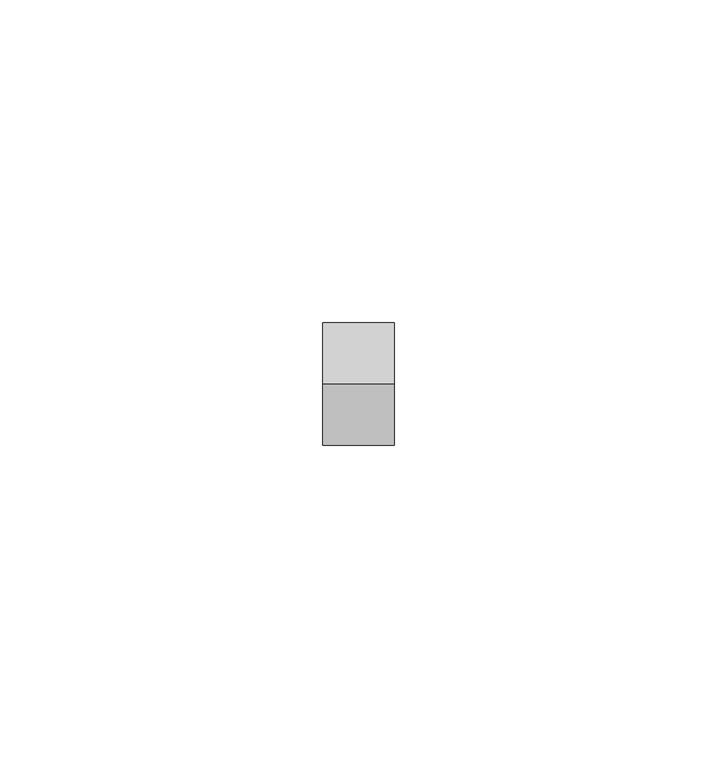
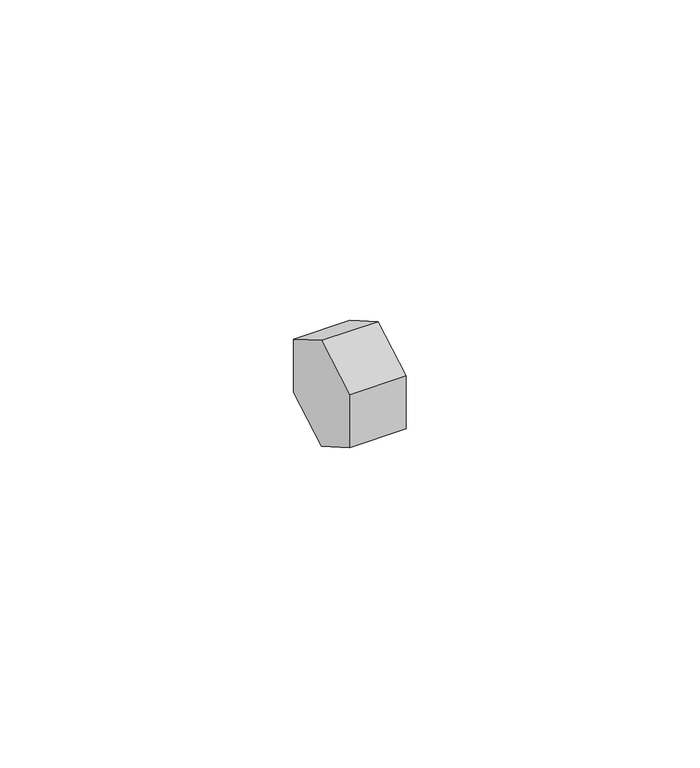
"""IFC4 building model written with IfcOpenShell, lengths in millimetres: proxy geometry, Generic Models 7:Generic Models 1:8:Generic Models 1:8 : Generic Models 7:Generic Models 1:337419:58 : Generic Models 7:Generic Models 1:8:Generic Models 1:8 : Generic Models 7:Generic Models 1:337419:315935."""

import ifcopenshell
import ifcopenshell.guid

model = None  # the IFC model being written
_history = None  # IfcOwnerHistory: only IFC2X3 demands one
_inside = {}  # id of a spatial element -> (the spatial element, [elements in it])
_under = {}  # id of a project, library or spatial element -> (it, [spatial elements below it])
_declared = {}  # id of a project -> (the project, [libraries it declares])
_typed = {}  # id of a type object -> (the type object, [elements of that type])
_made_of = {}  # id of a material, layer set ... -> (it, [elements and type objects made of it])


def new_model(schema):
    """Start an empty IFC model of exactly this schema.

    Asked for "IFC4X3", IfcOpenShell would pick the latest addendum, in which some entities
    have other attributes; the version numbers below select the first issue.
    IFC2X3 requires an IfcOwnerHistory on every rooted entity: one is made here for all.
    """
    global model, _history
    if schema == "IFC4X3":
        model = ifcopenshell.file(schema_version=(4, 3, 0, 0))
    else:
        model = ifcopenshell.file(schema=schema)
    _inside.clear()
    _under.clear()
    _declared.clear()
    _typed.clear()
    _made_of.clear()
    _history = None
    if model.schema == "IFC2X3":
        org = make("IfcOrganization", Name="unknown")
        user = make(
            "IfcPersonAndOrganization",
            ThePerson=make("IfcPerson", FamilyName="unknown"),
            TheOrganization=org,
        )
        app = make(
            "IfcApplication",
            ApplicationDeveloper=org,
            Version="unknown",
            ApplicationFullName="unknown",
            ApplicationIdentifier="unknown",
        )
        _history = make(
            "IfcOwnerHistory",
            OwningUser=user,
            OwningApplication=app,
            ChangeAction="ADDED",
            CreationDate=0,
        )
    return model


def make(cls, **values):
    """One entity of the class cls with the attributes given. An attribute that is None is left unset."""
    return model.create_entity(
        cls, **{name: value for name, value in values.items() if value is not None}
    )


def rooted(cls, **values):
    """An entity with a GlobalId (a new one), such as an element, a storey or a relation."""
    return make(cls, GlobalId=ifcopenshell.guid.new(), OwnerHistory=_history, **values)


def si_unit(unit_type, name, prefix=None):
    """IfcSIUnit, for example si_unit("LENGTHUNIT", "METRE", prefix="MILLI")."""
    return make("IfcSIUnit", UnitType=unit_type, Prefix=prefix, Name=name)


def assignment(units):
    """IfcUnitAssignment: the units of a project."""
    return None if units is None else make("IfcUnitAssignment", Units=units)


def point(xyz):
    """IfcCartesianPoint."""
    return None if xyz is None else make("IfcCartesianPoint", Coordinates=xyz)


def direction(xyz):
    """IfcDirection."""
    return None if xyz is None else make("IfcDirection", DirectionRatios=xyz)


def frame(location, z_axis=None, x_axis=None):
    """IfcAxis2Placement3D, a coordinate frame: its origin and axes. An axis left out is left unset."""
    return make(
        "IfcAxis2Placement3D",
        Location=point(location),
        Axis=direction(z_axis),
        RefDirection=direction(x_axis),
    )


def origin():
    """The frame at (0, 0, 0) with its axes left unset."""
    return frame((0.0, 0.0, 0.0))


def place(relative_to, where):
    """IfcLocalPlacement: puts the frame where relative to a parent placement (None: the world)."""
    return make(
        "IfcLocalPlacement", PlacementRelTo=relative_to, RelativePlacement=where
    )


def context(
    kind, dimensions, precision=None, world=None, true_north=None, identifier=None
):
    """IfcGeometricRepresentationContext, for example the 3D "Model" context."""
    return make(
        "IfcGeometricRepresentationContext",
        ContextIdentifier=identifier,
        ContextType=kind,
        CoordinateSpaceDimension=dimensions,
        Precision=precision,
        WorldCoordinateSystem=world,
        TrueNorth=true_north,
    )


def project(units=None, contexts=None):
    """IfcProject with its units and contexts."""
    return rooted(
        "IfcProject",
        Name="project",
        RepresentationContexts=contexts,
        UnitsInContext=assignment(units),
    )


def spatial(cls, under=None, at=None, **own):
    """A site, building, storey or space (cls), placed at a placement, below another one or the project."""
    s = rooted(cls, ObjectPlacement=at, **own)
    if under is not None:
        _under.setdefault(under.id(), (under, []))[1].append(s)
    return s


def polyline(points):
    """IfcPolyline through the points."""
    return make("IfcPolyline", Points=[point(p) for p in points])


def outline(outer, holes=None, kind="AREA"):
    """IfcArbitraryClosedProfileDef: a profile drawn as a closed curve; with holes, ...WithVoids."""
    if holes is None:
        return make("IfcArbitraryClosedProfileDef", ProfileType=kind, OuterCurve=outer)
    return make(
        "IfcArbitraryProfileDefWithVoids",
        ProfileType=kind,
        OuterCurve=outer,
        InnerCurves=holes,
    )


def extrude(swept, where, along, depth):
    """IfcExtrudedAreaSolid: the profile swept, set in the frame where, extruded along a direction by depth."""
    return make(
        "IfcExtrudedAreaSolid",
        SweptArea=swept,
        Position=where,
        ExtrudedDirection=direction(along),
        Depth=depth,
    )


def shape(context_of_items, identifier, shape_type, items):
    """IfcShapeRepresentation: the items that make up one representation, for example the "Body"."""
    return make(
        "IfcShapeRepresentation",
        ContextOfItems=context_of_items,
        RepresentationIdentifier=identifier,
        RepresentationType=shape_type,
        Items=items,
    )


def source(mapping_origin, context_of_items, identifier, shape_type, items):
    """IfcRepresentationMap: a shape defined once, which mapped items show again and again."""
    return make(
        "IfcRepresentationMap",
        MappingOrigin=mapping_origin,
        MappedRepresentation=shape(context_of_items, identifier, shape_type, items),
    )


def transform(
    local_origin,
    x_axis=None,
    y_axis=None,
    z_axis=None,
    scale=None,
    scale2=None,
    scale3=None,
    uniform=True,
):
    """IfcCartesianTransformationOperator3D, or its non-uniform kind. x_axis, y_axis, z_axis: its Axis1, 2, 3."""
    if uniform:
        return make(
            "IfcCartesianTransformationOperator3D",
            Axis1=direction(x_axis),
            Axis2=direction(y_axis),
            LocalOrigin=point(local_origin),
            Scale=scale,
            Axis3=direction(z_axis),
        )
    return make(
        "IfcCartesianTransformationOperator3DnonUniform",
        Axis1=direction(x_axis),
        Axis2=direction(y_axis),
        LocalOrigin=point(local_origin),
        Scale=scale,
        Axis3=direction(z_axis),
        Scale2=scale2,
        Scale3=scale3,
    )


def mapped(mapping_source, mapping_target):
    """IfcMappedItem: shows the shape of a source again, moved by a transform."""
    return make(
        "IfcMappedItem", MappingSource=mapping_source, MappingTarget=mapping_target
    )


def made_of(thing, what):
    """Note that an element or type object is made of a material, layer set ...; save() writes the relation."""
    if what is not None:
        _made_of.setdefault(what.id(), (what, []))[1].append(thing)
    return thing


def element(
    cls,
    number,
    at=None,
    inside=None,
    cuts=None,
    type_object=None,
    material=None,
    context=None,
    identifier="Body",
    shape_type=None,
    held_by="IfcProductDefinitionShape",
    body=None,
    shapes=None,
    **own,
):
    """One element of the class cls, such as IfcWall. Its Tag is "e" and its number.

    at: its placement. inside: the storey or other place that contains it. cuts: it is an
    opening in that element (IfcRelVoidsElement). A single representation is given by context,
    identifier, shape_type and body (its items); several are given by shapes. held_by: the class
    of the entity that holds the representations. save() writes the other relations.
    """
    e = rooted(cls, Tag="e%d" % number, ObjectPlacement=at, **own)
    if body is not None:
        shapes = [shape(context, identifier, shape_type, body)]
    if shapes is not None:
        e.Representation = make(held_by, Representations=shapes)
    if inside is not None:
        _inside.setdefault(inside.id(), (inside, []))[1].append(e)
    if cuts is not None:
        rooted(
            "IfcRelVoidsElement", RelatingBuildingElement=cuts, RelatedOpeningElement=e
        )
    if type_object is not None:
        _typed.setdefault(type_object.id(), (type_object, []))[1].append(e)
    return made_of(e, material)


def aggregate(whole, parts):
    """IfcRelAggregates: a whole, such as a stair, and the parts it consists of."""
    return rooted("IfcRelAggregates", RelatingObject=whole, RelatedObjects=parts)


def save(model, path):
    """Write the relations noted so far, then the file.

    IfcRelAggregates (storeys below a building ...), IfcRelContainedInSpatialStructure (elements
    in a storey), IfcRelDefinesByType, IfcRelAssociatesMaterial and IfcRelDeclares: one each for
    every whole, place, type object, material and project.
    """
    for whole, parts in _under.values():
        aggregate(whole, parts)
    for where, things in _inside.values():
        rooted(
            "IfcRelContainedInSpatialStructure",
            RelatedElements=things,
            RelatingStructure=where,
        )
    for kind, things in _typed.values():
        rooted("IfcRelDefinesByType", RelatedObjects=things, RelatingType=kind)
    for what, things in _made_of.values():
        rooted("IfcRelAssociatesMaterial", RelatedObjects=things, RelatingMaterial=what)
    for by, libraries in _declared.values():
        rooted("IfcRelDeclares", RelatingContext=by, RelatedDefinitions=libraries)
    model.write(path)


def generic_models_35fd506f(model_context):
    return source(origin(), model_context, "Body", "SweptSolid", [
        extrude(outline(polyline([(-564915.9326015, 8757.3782009), (-564925.4576015, 8762.8774622), (-564925.4576015, 8773.8759848), (-564915.9326015, 8779.3752461), (-564906.4076015, 8773.8759848), (-564906.4076015, 8762.8774622), (-564915.9326015, 8757.3782009)])), frame((593804.563286, 0.0, 0.0), z_axis=(1.0, 0.0, 0.0), x_axis=(0.0, 1.0, 0.0)), (0.0, 0.0, 1.0), 11.1125),
    ])


if __name__ == "__main__":
    model = new_model("IFC4")
    model_context = context("Model", 3, world=origin())
    ifc_project = project(units=[si_unit("LENGTHUNIT", "METRE", prefix="MILLI")], contexts=[model_context])
    site = spatial("IfcSite", under=ifc_project)
    building = spatial("IfcBuilding", under=site)
    placement = place(None, origin())
    generic_models_shape = generic_models_35fd506f(model_context)
    element("IfcBuildingElementProxy", 1, Name="Generic Models 7:Generic Models 1:8:Generic Models 1:8 : Generic Models 7:Generic Models 1:337419:58 : Generic Models 7:Generic Models 1:8:Generic Models 1:8 : Generic Models 7:Generic Models 1:337419:315935", ObjectType="Generic Models 7:Generic Models 1:8:Generic Models 1:8 : Generic Models 7:Generic Models 1:337419:58 : Generic Models 7:Generic Models 1:8:Generic Models 1:8 : Generic Models 7:Generic Models 1:337419:315935", at=placement, inside=building, context=model_context, shape_type="MappedRepresentation", body=[
        mapped(generic_models_shape, transform((0.0, 0.0, 0.0), x_axis=(1.0, 0.0, 0.0), y_axis=(0.0, 1.0, 0.0), z_axis=(0.0, 0.0, 1.0))),
    ])
    save(model, "model.ifc")

# Revit data of these elements
# Type "Generic Models 7:Generic Models 1:8:Generic Models 1:8 : Generic Models 7:Generic Models 1:337419:58 : Generic Models 7:Generic Models 1:8:Generic Models 1:8 : Generic Models 7:Generic Models 1:337419:315935"
#   NameOverride = "Generic Models 7:Generic Models 1:8:Generic Models 1:8 : Generic Models 7:Generic Models 1:337419:315935"
#   ObjectTypeOverride = "Generic Models 1:8 : Generic Models 7:Generic Models 1:337419"
#   Reference = "Generic Models 1"
#   Tag = "315935"
# Element 1 (IfcBuildingElementProxy, "Generic Models 7:Generic Models 1:8:Generic Models 1:8 : Generic Models 7:Generic Models 1:337419:58 : Generic Models 7:Generic Models 1:8:Generic Models 1:8 : Generic Models 7:Generic Models 1:337419:315935")
#   Materials on its faces: "1/2\" THRU BOLTS"
# Materials
#   "1/2\" THRU BOLTS": class "Generic", colour RGB 120 120 120, transparency 0, Cost = 0
